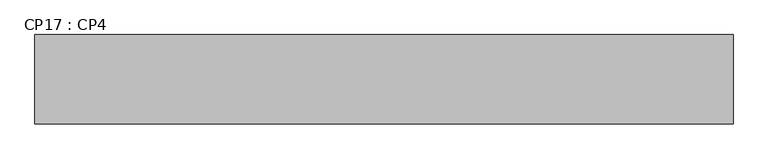
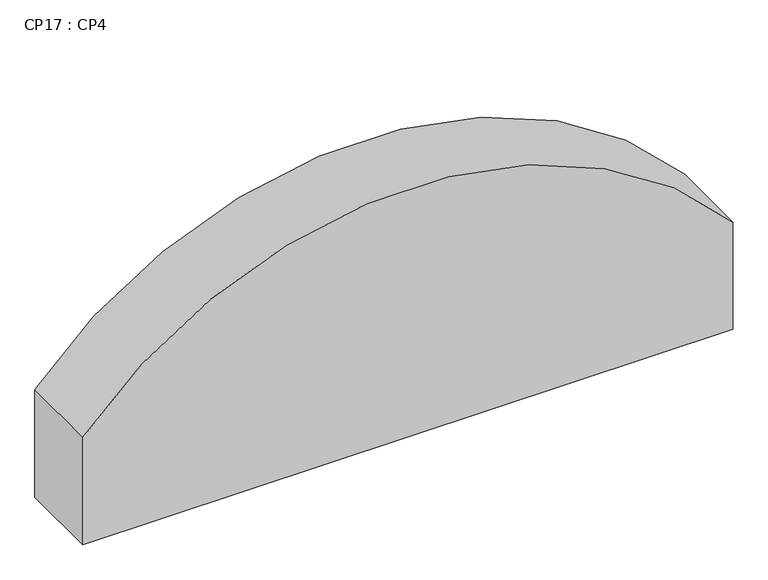
"""IFC4 building model written with IfcOpenShell, lengths in millimetres: beam geometry, CP17 : CP4."""

import ifcopenshell
import ifcopenshell.guid

model = None  # the IFC model being written
_history = None  # IfcOwnerHistory: only IFC2X3 demands one
_inside = {}  # id of a spatial element -> (the spatial element, [elements in it])
_under = {}  # id of a project, library or spatial element -> (it, [spatial elements below it])
_declared = {}  # id of a project -> (the project, [libraries it declares])
_typed = {}  # id of a type object -> (the type object, [elements of that type])
_made_of = {}  # id of a material, layer set ... -> (it, [elements and type objects made of it])


def new_model(schema):
    """Start an empty IFC model of exactly this schema.

    Asked for "IFC4X3", IfcOpenShell would pick the latest addendum, in which some entities
    have other attributes; the version numbers below select the first issue.
    IFC2X3 requires an IfcOwnerHistory on every rooted entity: one is made here for all.
    """
    global model, _history
    if schema == "IFC4X3":
        model = ifcopenshell.file(schema_version=(4, 3, 0, 0))
    else:
        model = ifcopenshell.file(schema=schema)
    _inside.clear()
    _under.clear()
    _declared.clear()
    _typed.clear()
    _made_of.clear()
    _history = None
    if model.schema == "IFC2X3":
        org = make("IfcOrganization", Name="unknown")
        user = make(
            "IfcPersonAndOrganization",
            ThePerson=make("IfcPerson", FamilyName="unknown"),
            TheOrganization=org,
        )
        app = make(
            "IfcApplication",
            ApplicationDeveloper=org,
            Version="unknown",
            ApplicationFullName="unknown",
            ApplicationIdentifier="unknown",
        )
        _history = make(
            "IfcOwnerHistory",
            OwningUser=user,
            OwningApplication=app,
            ChangeAction="ADDED",
            CreationDate=0,
        )
    return model


def make(cls, **values):
    """One entity of the class cls with the attributes given. An attribute that is None is left unset."""
    return model.create_entity(
        cls, **{name: value for name, value in values.items() if value is not None}
    )


def rooted(cls, **values):
    """An entity with a GlobalId (a new one), such as an element, a storey or a relation."""
    return make(cls, GlobalId=ifcopenshell.guid.new(), OwnerHistory=_history, **values)


def si_unit(unit_type, name, prefix=None):
    """IfcSIUnit, for example si_unit("LENGTHUNIT", "METRE", prefix="MILLI")."""
    return make("IfcSIUnit", UnitType=unit_type, Prefix=prefix, Name=name)


def assignment(units):
    """IfcUnitAssignment: the units of a project."""
    return None if units is None else make("IfcUnitAssignment", Units=units)


def point(xyz):
    """IfcCartesianPoint."""
    return None if xyz is None else make("IfcCartesianPoint", Coordinates=xyz)


def direction(xyz):
    """IfcDirection."""
    return None if xyz is None else make("IfcDirection", DirectionRatios=xyz)


def frame(location, z_axis=None, x_axis=None):
    """IfcAxis2Placement3D, a coordinate frame: its origin and axes. An axis left out is left unset."""
    return make(
        "IfcAxis2Placement3D",
        Location=point(location),
        Axis=direction(z_axis),
        RefDirection=direction(x_axis),
    )


def origin():
    """The frame at (0, 0, 0) with its axes left unset."""
    return frame((0.0, 0.0, 0.0))


def place(relative_to, where):
    """IfcLocalPlacement: puts the frame where relative to a parent placement (None: the world)."""
    return make(
        "IfcLocalPlacement", PlacementRelTo=relative_to, RelativePlacement=where
    )


def context(
    kind, dimensions, precision=None, world=None, true_north=None, identifier=None
):
    """IfcGeometricRepresentationContext, for example the 3D "Model" context."""
    return make(
        "IfcGeometricRepresentationContext",
        ContextIdentifier=identifier,
        ContextType=kind,
        CoordinateSpaceDimension=dimensions,
        Precision=precision,
        WorldCoordinateSystem=world,
        TrueNorth=true_north,
    )


def project(units=None, contexts=None):
    """IfcProject with its units and contexts."""
    return rooted(
        "IfcProject",
        Name="project",
        RepresentationContexts=contexts,
        UnitsInContext=assignment(units),
    )


def spatial(cls, under=None, at=None, **own):
    """A site, building, storey or space (cls), placed at a placement, below another one or the project."""
    s = rooted(cls, ObjectPlacement=at, **own)
    if under is not None:
        _under.setdefault(under.id(), (under, []))[1].append(s)
    return s


def circle_curve(where, radius):
    """IfcCircle in the frame where."""
    return make("IfcCircle", Position=where, Radius=radius)


def shape(context_of_items, identifier, shape_type, items):
    """IfcShapeRepresentation: the items that make up one representation, for example the "Body"."""
    return make(
        "IfcShapeRepresentation",
        ContextOfItems=context_of_items,
        RepresentationIdentifier=identifier,
        RepresentationType=shape_type,
        Items=items,
    )


def source(mapping_origin, context_of_items, identifier, shape_type, items):
    """IfcRepresentationMap: a shape defined once, which mapped items show again and again."""
    return make(
        "IfcRepresentationMap",
        MappingOrigin=mapping_origin,
        MappedRepresentation=shape(context_of_items, identifier, shape_type, items),
    )


def transform(
    local_origin,
    x_axis=None,
    y_axis=None,
    z_axis=None,
    scale=None,
    scale2=None,
    scale3=None,
    uniform=True,
):
    """IfcCartesianTransformationOperator3D, or its non-uniform kind. x_axis, y_axis, z_axis: its Axis1, 2, 3."""
    if uniform:
        return make(
            "IfcCartesianTransformationOperator3D",
            Axis1=direction(x_axis),
            Axis2=direction(y_axis),
            LocalOrigin=point(local_origin),
            Scale=scale,
            Axis3=direction(z_axis),
        )
    return make(
        "IfcCartesianTransformationOperator3DnonUniform",
        Axis1=direction(x_axis),
        Axis2=direction(y_axis),
        LocalOrigin=point(local_origin),
        Scale=scale,
        Axis3=direction(z_axis),
        Scale2=scale2,
        Scale3=scale3,
    )


def mapped(mapping_source, mapping_target):
    """IfcMappedItem: shows the shape of a source again, moved by a transform."""
    return make(
        "IfcMappedItem", MappingSource=mapping_source, MappingTarget=mapping_target
    )


def made_of(thing, what):
    """Note that an element or type object is made of a material, layer set ...; save() writes the relation."""
    if what is not None:
        _made_of.setdefault(what.id(), (what, []))[1].append(thing)
    return thing


def element(
    cls,
    number,
    at=None,
    inside=None,
    cuts=None,
    type_object=None,
    material=None,
    context=None,
    identifier="Body",
    shape_type=None,
    held_by="IfcProductDefinitionShape",
    body=None,
    shapes=None,
    **own,
):
    """One element of the class cls, such as IfcWall. Its Tag is "e" and its number.

    at: its placement. inside: the storey or other place that contains it. cuts: it is an
    opening in that element (IfcRelVoidsElement). A single representation is given by context,
    identifier, shape_type and body (its items); several are given by shapes. held_by: the class
    of the entity that holds the representations. save() writes the other relations.
    """
    e = rooted(cls, Tag="e%d" % number, ObjectPlacement=at, **own)
    if body is not None:
        shapes = [shape(context, identifier, shape_type, body)]
    if shapes is not None:
        e.Representation = make(held_by, Representations=shapes)
    if inside is not None:
        _inside.setdefault(inside.id(), (inside, []))[1].append(e)
    if cuts is not None:
        rooted(
            "IfcRelVoidsElement", RelatingBuildingElement=cuts, RelatedOpeningElement=e
        )
    if type_object is not None:
        _typed.setdefault(type_object.id(), (type_object, []))[1].append(e)
    return made_of(e, material)


def aggregate(whole, parts):
    """IfcRelAggregates: a whole, such as a stair, and the parts it consists of."""
    return rooted("IfcRelAggregates", RelatingObject=whole, RelatedObjects=parts)


def save(model, path):
    """Write the relations noted so far, then the file.

    IfcRelAggregates (storeys below a building ...), IfcRelContainedInSpatialStructure (elements
    in a storey), IfcRelDefinesByType, IfcRelAssociatesMaterial and IfcRelDeclares: one each for
    every whole, place, type object, material and project.
    """
    for whole, parts in _under.values():
        aggregate(whole, parts)
    for where, things in _inside.values():
        rooted(
            "IfcRelContainedInSpatialStructure",
            RelatedElements=things,
            RelatingStructure=where,
        )
    for kind, things in _typed.values():
        rooted("IfcRelDefinesByType", RelatedObjects=things, RelatingType=kind)
    for what, things in _made_of.values():
        rooted("IfcRelAssociatesMaterial", RelatedObjects=things, RelatingMaterial=what)
    for by, libraries in _declared.values():
        rooted("IfcRelDeclares", RelatingContext=by, RelatedDefinitions=libraries)
    model.write(path)


def plane_surface(at):
    """IfcPlane: the flat surface through the origin of the frame at, square to its z axis."""
    return make("IfcPlane", Position=at)


def cylinder_surface(at, radius):
    """IfcCylindricalSurface: all points at the distance radius from the z axis of the frame at."""
    return make("IfcCylindricalSurface", Position=at, Radius=radius)


def advanced_brep(points, edges, surfaces, faces):
    """IfcAdvancedBrep: a solid bounded by faces that lie on surfaces and meet in shared edges.

    An edge is (start, end): straight between two places in points (the first is 0);
    or (start, end, curve); or (start, end, curve, False) where it runs against its curve.
    A face is (place in surfaces, loops), or (place, loops, False) where it looks against
    its surface's normal. A loop lists edges by number (the first is 1), with a minus sign
    where the edge is run from its end to its start. The first loop is the outer one.
    """
    corners = [point(p) for p in points]
    vertices = [make("IfcVertexPoint", VertexGeometry=c) for c in corners]
    made = []
    for start, end, *more in edges:
        made.append(
            make(
                "IfcEdgeCurve",
                EdgeStart=vertices[start],
                EdgeEnd=vertices[end],
                EdgeGeometry=more[0] if more else make("IfcPolyline", Points=[corners[start], corners[end]]),
                SameSense=more[1] if len(more) > 1 else True,
            )
        )
    hull = []
    for where, loops, *sense in faces:
        bounds = []
        for j, loop in enumerate(loops):
            ring = [make("IfcOrientedEdge", EdgeElement=made[abs(k) - 1], Orientation=k > 0) for k in loop]
            bounds.append(
                make(
                    "IfcFaceOuterBound" if j == 0 else "IfcFaceBound",
                    Bound=make("IfcEdgeLoop", EdgeList=ring),
                    Orientation=True,
                )
            )
        hull.append(make("IfcAdvancedFace", Bounds=bounds, FaceSurface=surfaces[where], SameSense=sense[0] if sense else True))
    return make("IfcAdvancedBrep", Outer=make("IfcClosedShell", CfsFaces=hull))


def cp17_cp4_f2bb5386(model_context):
    return source(origin(), model_context, "Body", "AdvancedBrep", [
        advanced_brep(
        [(5143.2245516, 20099.7448193, 13800.0), (5143.2245516, 20099.7448193, 14620.0), (9843.2245541, 20099.7448193, 14620.0), (9843.2245521, 20099.7448193, 13800.0), (9843.2245541, 19499.6999972, 14620.0), (5143.2245542, 19499.6999972, 14620.0), (5143.2245516, 19499.6999972, 13800.0), (9843.2245521, 19499.6999972, 13800.0)],
        [
            (0, 1),
            (1, 2, circle_curve(frame((7493.2245542, 20099.7448193, 12603.2870371), z_axis=(0.0, 1.0, 0.0), x_axis=(0.0, 0.0, -1.0)), 3096.7129629)),
            (2, 3),
            (3, 0),
            (4, 5, circle_curve(frame((7493.2245542, 19499.6999972, 12603.2870371), z_axis=(0.0, -1.0, 0.0), x_axis=(0.0, 0.0, -1.0)), 3096.7129629)),
            (5, 6),
            (6, 7),
            (7, 4),
            (6, 0),
            (3, 7),
            (4, 2),
            (1, 5),
        ],
        [
            plane_surface(frame((7493.2245542, 20099.7448193, 9323.3898307), z_axis=(0.0, 1.0, 0.0), x_axis=(-1.0, 0.0, 0.0))),
            plane_surface(frame((7493.2245542, 19499.6999972, 9323.3898307), z_axis=(0.0, -1.0, 0.0), x_axis=(1.0, 0.0, 0.0))),
            plane_surface(frame((9993.2245541, 20099.7448193, 13800.0), z_axis=(0.0, 0.0, -1.0), x_axis=(0.0, -1.0, 0.0))),
            cylinder_surface(frame((7493.2245542, 20099.7448193, 12603.2870371), z_axis=(0.0, 1.0, 0.0), x_axis=(0.0, 0.0, -1.0)), 3096.7129629),
            plane_surface(frame((5143.2245516, 18587.0448193, 14620.0), z_axis=(-1.0, 0.0, 0.0), x_axis=(0.0, -1.0, 0.0))),
            plane_surface(frame((9843.2245521, 18587.0448193, 13800.0), z_axis=(1.0, 0.0, 0.0), x_axis=(0.0, -1.0, 0.0))),
        ],
        [
            (0, [[1, 2, 3, 4]]),
            (1, [[5, 6, 7, 8]]),
            (2, [[9, -4, 10, -7]]),
            (3, [[-5, 11, -2, 12]]),
            (4, [[-1, -9, -6, -12]]),
            (5, [[-3, -11, -8, -10]]),
        ],
    ),
    ])


if __name__ == "__main__":
    model = new_model("IFC4")
    model_context = context("Model", 3, world=origin())
    ifc_project = project(units=[si_unit("LENGTHUNIT", "METRE", prefix="MILLI")], contexts=[model_context])
    site = spatial("IfcSite", under=ifc_project)
    building = spatial("IfcBuilding", under=site)
    placement = place(None, origin())
    cp17_cp4_shape = cp17_cp4_f2bb5386(model_context)
    element("IfcBeam", 1, ObjectType="CP17 : CP4", at=placement, inside=building, context=model_context, shape_type="MappedRepresentation", body=[
        mapped(cp17_cp4_shape, transform((0.0, 0.0, 0.0), x_axis=(1.0, 0.0, 0.0), y_axis=(0.0, 1.0, 0.0), z_axis=(0.0, 0.0, 1.0))),
    ])
    save(model, "model.ifc")
